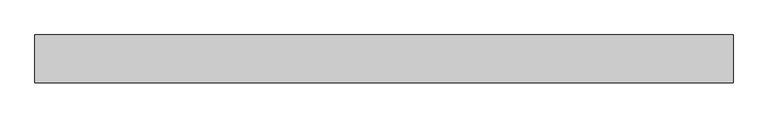
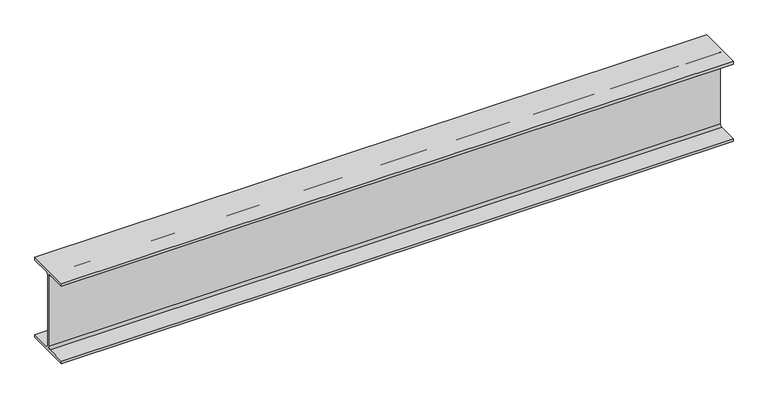
"""IFC4 building model written with IfcOpenShell, lengths in millimetres: beam geometry, Old_Steel Beam_H-KSD3502 : H_SB_ASB_H-200×200x8x12."""

from ifc_helpers import new_model, si_unit, point, frame, frame_2d, origin, place, context, project, spatial, polyline, circle_curve, trimmed, segment, composite_curve, outline, extrude, source, transform, mapped, element, save


def beam_92807fc5(model_context):
    return source(origin(), model_context, "Body", "SweptSolid", [
        extrude(outline(composite_curve([segment(polyline([(82.5, -141.5), (82.5, -151.7), (-82.5, -151.7), (-82.5, -141.5), (-11.9, -141.5)]), True, "CONTINUOUS"), segment(trimmed(circle_curve(frame_2d((-11.9, -132.6)), 8.9), [point((-11.9, -141.5))], [point((-3.0, -132.6))], True, "CARTESIAN"), True, "CONTINUOUS"), segment(polyline([(-3.0, -132.6), (-3.0, 132.6)]), True, "CONTINUOUS"), segment(trimmed(circle_curve(frame_2d((-11.9, 132.6)), 8.9), [point((-3.0, 132.6))], [point((-11.9, 141.5))], True, "CARTESIAN"), True, "CONTINUOUS"), segment(polyline([(-11.9, 141.5), (-82.5, 141.5), (-82.5, 151.7), (82.5, 151.7), (82.5, 141.5), (11.9, 141.5)]), True, "CONTINUOUS"), segment(trimmed(circle_curve(frame_2d((11.9, 132.6)), 8.9), [point((11.9, 141.5))], [point((3.0, 132.6))], True, "CARTESIAN"), True, "CONTINUOUS"), segment(polyline([(3.0, 132.6), (3.0, -132.6)]), True, "CONTINUOUS"), segment(trimmed(circle_curve(frame_2d((11.9, -132.6)), 8.9), [point((3.0, -132.6))], [point((11.9, -141.5))], True, "CARTESIAN"), True, "CONTINUOUS"), segment(polyline([(11.9, -141.5), (82.5, -141.5)]), True, "CONTINUOUS")], self_intersect=False)), frame((-1199.8807155, 0.0, 0.0), z_axis=(1.0, 0.0, 0.0), x_axis=(0.0, 1.0, 0.0)), (0.0, 0.0, 1.0), 2406.4861403),
    ])


if __name__ == "__main__":
    model = new_model("IFC4")
    model_context = context("Model", 3, world=origin())
    ifc_project = project(units=[si_unit("LENGTHUNIT", "METRE", prefix="MILLI")], contexts=[model_context])
    site = spatial("IfcSite", under=ifc_project)
    building = spatial("IfcBuilding", under=site)
    placement = place(None, origin())
    beam_shape = beam_92807fc5(model_context)
    element("IfcBeam", 1, ObjectType="Old_Steel Beam_H-KSD3502 : H_SB_ASB_H-200×200x8x12", at=placement, inside=building, context=model_context, shape_type="MappedRepresentation", body=[
        mapped(beam_shape, transform((0.0, 0.0, 0.0), x_axis=(1.0, 0.0, 0.0), y_axis=(0.0, 1.0, 0.0), z_axis=(0.0, 0.0, 1.0))),
    ])
    save(model, "model.ifc")

# Revit data of these elements
# Type "Old_Steel Beam_H-KSD3502 : H_SB_ASB_H-200×200x8x12"
#   Width = 20.0 cm
#   Web Thickness = 0.8 cm
#   Web Fillet = 1.3 cm
#   Warping Constant = 141376.0 cm⁶
#   Torsional Moment of Inertia = 26.2485 cm⁴
#   Torsional Modulus = 1.0 cm³
#   Section Area = 63.53 cm²
#   Plastic Modulus weak axis = 244.0 cm³
#   Plastic Modulus strong axis = 525.0 cm³
#   Perimeter = 1.16 m²/m
#   Nominal Weight = 49.90 kgf/m
#   Moment of Inertia weak axis = 1600.00 cm⁴
#   Moment of Inertia strong axis = 4720.00 cm⁴
#   Height = 20.0 cm
#   Flange Thickness = 1.2 cm
#   Elastic Modulus weak axis = 160.0 cm³
#   Elastic Modulus strong axis = 472.0 cm³
#   Centroid Vertical = 10.0 cm
#   Centroid Horizontal = 10.0 cm
#   Length [instance default] = 1.5240 m
#   Structural Material [instance default] = Steel, 45-345
#   Assembly Code = ""
# Element 1 (IfcBeam, "Old_Steel Beam_H-KSD3502 : H_SB_ASB_H-200×200x8x12")
#   Structural Material = none
# Materials
#   "Steel, 45-345": class "Metal", colour RGB 189 187 185, transparency 0, Description = "Steel 345 MPa", Cost = 0
